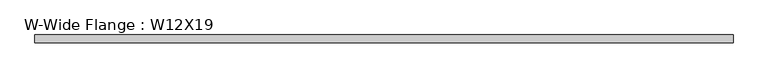
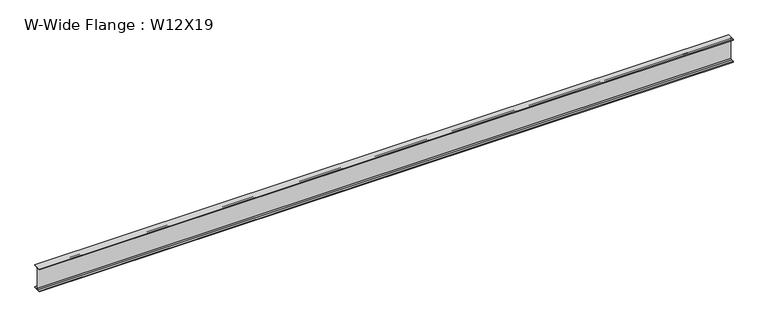
"""IFC4 building model written with IfcOpenShell, lengths in millimetres: beam geometry, W-Wide Flange : W12X19."""

import ifcopenshell
import ifcopenshell.guid

model = None  # the IFC model being written
_history = None  # IfcOwnerHistory: only IFC2X3 demands one
_inside = {}  # id of a spatial element -> (the spatial element, [elements in it])
_under = {}  # id of a project, library or spatial element -> (it, [spatial elements below it])
_declared = {}  # id of a project -> (the project, [libraries it declares])
_typed = {}  # id of a type object -> (the type object, [elements of that type])
_made_of = {}  # id of a material, layer set ... -> (it, [elements and type objects made of it])


def new_model(schema):
    """Start an empty IFC model of exactly this schema.

    Asked for "IFC4X3", IfcOpenShell would pick the latest addendum, in which some entities
    have other attributes; the version numbers below select the first issue.
    IFC2X3 requires an IfcOwnerHistory on every rooted entity: one is made here for all.
    """
    global model, _history
    if schema == "IFC4X3":
        model = ifcopenshell.file(schema_version=(4, 3, 0, 0))
    else:
        model = ifcopenshell.file(schema=schema)
    _inside.clear()
    _under.clear()
    _declared.clear()
    _typed.clear()
    _made_of.clear()
    _history = None
    if model.schema == "IFC2X3":
        org = make("IfcOrganization", Name="unknown")
        user = make(
            "IfcPersonAndOrganization",
            ThePerson=make("IfcPerson", FamilyName="unknown"),
            TheOrganization=org,
        )
        app = make(
            "IfcApplication",
            ApplicationDeveloper=org,
            Version="unknown",
            ApplicationFullName="unknown",
            ApplicationIdentifier="unknown",
        )
        _history = make(
            "IfcOwnerHistory",
            OwningUser=user,
            OwningApplication=app,
            ChangeAction="ADDED",
            CreationDate=0,
        )
    return model


def make(cls, **values):
    """One entity of the class cls with the attributes given. An attribute that is None is left unset."""
    return model.create_entity(
        cls, **{name: value for name, value in values.items() if value is not None}
    )


def rooted(cls, **values):
    """An entity with a GlobalId (a new one), such as an element, a storey or a relation."""
    return make(cls, GlobalId=ifcopenshell.guid.new(), OwnerHistory=_history, **values)


def si_unit(unit_type, name, prefix=None):
    """IfcSIUnit, for example si_unit("LENGTHUNIT", "METRE", prefix="MILLI")."""
    return make("IfcSIUnit", UnitType=unit_type, Prefix=prefix, Name=name)


def assignment(units):
    """IfcUnitAssignment: the units of a project."""
    return None if units is None else make("IfcUnitAssignment", Units=units)


def point(xyz):
    """IfcCartesianPoint."""
    return None if xyz is None else make("IfcCartesianPoint", Coordinates=xyz)


def direction(xyz):
    """IfcDirection."""
    return None if xyz is None else make("IfcDirection", DirectionRatios=xyz)


def frame(location, z_axis=None, x_axis=None):
    """IfcAxis2Placement3D, a coordinate frame: its origin and axes. An axis left out is left unset."""
    return make(
        "IfcAxis2Placement3D",
        Location=point(location),
        Axis=direction(z_axis),
        RefDirection=direction(x_axis),
    )


def frame_2d(location, x_axis=None):
    """IfcAxis2Placement2D, a coordinate frame in the plane: its origin and x axis."""
    return make(
        "IfcAxis2Placement2D", Location=point(location), RefDirection=direction(x_axis)
    )


def origin():
    """The frame at (0, 0, 0) with its axes left unset."""
    return frame((0.0, 0.0, 0.0))


def place(relative_to, where):
    """IfcLocalPlacement: puts the frame where relative to a parent placement (None: the world)."""
    return make(
        "IfcLocalPlacement", PlacementRelTo=relative_to, RelativePlacement=where
    )


def context(
    kind, dimensions, precision=None, world=None, true_north=None, identifier=None
):
    """IfcGeometricRepresentationContext, for example the 3D "Model" context."""
    return make(
        "IfcGeometricRepresentationContext",
        ContextIdentifier=identifier,
        ContextType=kind,
        CoordinateSpaceDimension=dimensions,
        Precision=precision,
        WorldCoordinateSystem=world,
        TrueNorth=true_north,
    )


def project(units=None, contexts=None):
    """IfcProject with its units and contexts."""
    return rooted(
        "IfcProject",
        Name="project",
        RepresentationContexts=contexts,
        UnitsInContext=assignment(units),
    )


def spatial(cls, under=None, at=None, **own):
    """A site, building, storey or space (cls), placed at a placement, below another one or the project."""
    s = rooted(cls, ObjectPlacement=at, **own)
    if under is not None:
        _under.setdefault(under.id(), (under, []))[1].append(s)
    return s


def polyline(points):
    """IfcPolyline through the points."""
    return make("IfcPolyline", Points=[point(p) for p in points])


def circle_curve(where, radius):
    """IfcCircle in the frame where."""
    return make("IfcCircle", Position=where, Radius=radius)


def trimmed(basis, trim1, trim2, sense, master):
    """IfcTrimmedCurve: the piece of a basis curve between two trims."""
    return make(
        "IfcTrimmedCurve",
        BasisCurve=basis,
        Trim1=trim1,
        Trim2=trim2,
        SenseAgreement=sense,
        MasterRepresentation=master,
    )


def segment(curve, same_sense, transition):
    """IfcCompositeCurveSegment."""
    return make(
        "IfcCompositeCurveSegment",
        Transition=transition,
        SameSense=same_sense,
        ParentCurve=curve,
    )


def composite_curve(segments, self_intersect=None):
    """IfcCompositeCurve: segments joined end to end."""
    return make("IfcCompositeCurve", Segments=segments, SelfIntersect=self_intersect)


def outline(outer, holes=None, kind="AREA"):
    """IfcArbitraryClosedProfileDef: a profile drawn as a closed curve; with holes, ...WithVoids."""
    if holes is None:
        return make("IfcArbitraryClosedProfileDef", ProfileType=kind, OuterCurve=outer)
    return make(
        "IfcArbitraryProfileDefWithVoids",
        ProfileType=kind,
        OuterCurve=outer,
        InnerCurves=holes,
    )


def extrude(swept, where, along, depth):
    """IfcExtrudedAreaSolid: the profile swept, set in the frame where, extruded along a direction by depth."""
    return make(
        "IfcExtrudedAreaSolid",
        SweptArea=swept,
        Position=where,
        ExtrudedDirection=direction(along),
        Depth=depth,
    )


def shape(context_of_items, identifier, shape_type, items):
    """IfcShapeRepresentation: the items that make up one representation, for example the "Body"."""
    return make(
        "IfcShapeRepresentation",
        ContextOfItems=context_of_items,
        RepresentationIdentifier=identifier,
        RepresentationType=shape_type,
        Items=items,
    )


def source(mapping_origin, context_of_items, identifier, shape_type, items):
    """IfcRepresentationMap: a shape defined once, which mapped items show again and again."""
    return make(
        "IfcRepresentationMap",
        MappingOrigin=mapping_origin,
        MappedRepresentation=shape(context_of_items, identifier, shape_type, items),
    )


def transform(
    local_origin,
    x_axis=None,
    y_axis=None,
    z_axis=None,
    scale=None,
    scale2=None,
    scale3=None,
    uniform=True,
):
    """IfcCartesianTransformationOperator3D, or its non-uniform kind. x_axis, y_axis, z_axis: its Axis1, 2, 3."""
    if uniform:
        return make(
            "IfcCartesianTransformationOperator3D",
            Axis1=direction(x_axis),
            Axis2=direction(y_axis),
            LocalOrigin=point(local_origin),
            Scale=scale,
            Axis3=direction(z_axis),
        )
    return make(
        "IfcCartesianTransformationOperator3DnonUniform",
        Axis1=direction(x_axis),
        Axis2=direction(y_axis),
        LocalOrigin=point(local_origin),
        Scale=scale,
        Axis3=direction(z_axis),
        Scale2=scale2,
        Scale3=scale3,
    )


def mapped(mapping_source, mapping_target):
    """IfcMappedItem: shows the shape of a source again, moved by a transform."""
    return make(
        "IfcMappedItem", MappingSource=mapping_source, MappingTarget=mapping_target
    )


def made_of(thing, what):
    """Note that an element or type object is made of a material, layer set ...; save() writes the relation."""
    if what is not None:
        _made_of.setdefault(what.id(), (what, []))[1].append(thing)
    return thing


def element(
    cls,
    number,
    at=None,
    inside=None,
    cuts=None,
    type_object=None,
    material=None,
    context=None,
    identifier="Body",
    shape_type=None,
    held_by="IfcProductDefinitionShape",
    body=None,
    shapes=None,
    **own,
):
    """One element of the class cls, such as IfcWall. Its Tag is "e" and its number.

    at: its placement. inside: the storey or other place that contains it. cuts: it is an
    opening in that element (IfcRelVoidsElement). A single representation is given by context,
    identifier, shape_type and body (its items); several are given by shapes. held_by: the class
    of the entity that holds the representations. save() writes the other relations.
    """
    e = rooted(cls, Tag="e%d" % number, ObjectPlacement=at, **own)
    if body is not None:
        shapes = [shape(context, identifier, shape_type, body)]
    if shapes is not None:
        e.Representation = make(held_by, Representations=shapes)
    if inside is not None:
        _inside.setdefault(inside.id(), (inside, []))[1].append(e)
    if cuts is not None:
        rooted(
            "IfcRelVoidsElement", RelatingBuildingElement=cuts, RelatedOpeningElement=e
        )
    if type_object is not None:
        _typed.setdefault(type_object.id(), (type_object, []))[1].append(e)
    return made_of(e, material)


def aggregate(whole, parts):
    """IfcRelAggregates: a whole, such as a stair, and the parts it consists of."""
    return rooted("IfcRelAggregates", RelatingObject=whole, RelatedObjects=parts)


def save(model, path):
    """Write the relations noted so far, then the file.

    IfcRelAggregates (storeys below a building ...), IfcRelContainedInSpatialStructure (elements
    in a storey), IfcRelDefinesByType, IfcRelAssociatesMaterial and IfcRelDeclares: one each for
    every whole, place, type object, material and project.
    """
    for whole, parts in _under.values():
        aggregate(whole, parts)
    for where, things in _inside.values():
        rooted(
            "IfcRelContainedInSpatialStructure",
            RelatedElements=things,
            RelatingStructure=where,
        )
    for kind, things in _typed.values():
        rooted("IfcRelDefinesByType", RelatedObjects=things, RelatingType=kind)
    for what, things in _made_of.values():
        rooted("IfcRelAssociatesMaterial", RelatedObjects=things, RelatingMaterial=what)
    for by, libraries in _declared.values():
        rooted("IfcRelDeclares", RelatingContext=by, RelatedDefinitions=libraries)
    model.write(path)


def w_wide_flange_w12x19_d63bb9e0(model_context):
    return source(origin(), model_context, "Body", "SweptSolid", [
        extrude(outline(composite_curve([segment(polyline([(50.927, -146.05), (50.927, -154.94), (-50.927, -154.94), (-50.927, -146.05), (-16.3195, -146.05)]), True, "CONTINUOUS"), segment(trimmed(circle_curve(frame_2d((-16.3195, -132.715)), 13.335), [point((-16.3195, -146.05))], [point((-2.9845, -132.715))], True, "CARTESIAN"), True, "CONTINUOUS"), segment(polyline([(-2.9845, -132.715), (-2.9845, 132.715)]), True, "CONTINUOUS"), segment(trimmed(circle_curve(frame_2d((-16.3195, 132.715)), 13.335), [point((-2.9845, 132.715))], [point((-16.3195, 146.05))], True, "CARTESIAN"), True, "CONTINUOUS"), segment(polyline([(-16.3195, 146.05), (-50.927, 146.05), (-50.927, 154.94), (50.927, 154.94), (50.927, 146.05), (16.3195, 146.05)]), True, "CONTINUOUS"), segment(trimmed(circle_curve(frame_2d((16.3195, 132.715)), 13.335), [point((16.3195, 146.05))], [point((2.9845, 132.715))], True, "CARTESIAN"), True, "CONTINUOUS"), segment(polyline([(2.9845, 132.715), (2.9845, -132.715)]), True, "CONTINUOUS"), segment(trimmed(circle_curve(frame_2d((16.3195, -132.715)), 13.335), [point((2.9845, -132.715))], [point((16.3195, -146.05))], True, "CARTESIAN"), True, "CONTINUOUS"), segment(polyline([(16.3195, -146.05), (50.927, -146.05)]), True, "CONTINUOUS")], self_intersect=False)), frame((-4381.4503906, 0.0, 0.0), z_axis=(1.0, 0.0, 0.0), x_axis=(0.0, 1.0, 0.0)), (0.0, 0.0, 1.0), 8953.4503906),
    ])


if __name__ == "__main__":
    model = new_model("IFC4")
    model_context = context("Model", 3, world=origin())
    ifc_project = project(units=[si_unit("LENGTHUNIT", "METRE", prefix="MILLI")], contexts=[model_context])
    site = spatial("IfcSite", under=ifc_project)
    building = spatial("IfcBuilding", under=site)
    placement = place(None, origin())
    w_wide_flange_w12x19_shape = w_wide_flange_w12x19_d63bb9e0(model_context)
    element("IfcBeam", 1, ObjectType="W-Wide Flange : W12X19", at=placement, inside=building, context=model_context, shape_type="MappedRepresentation", body=[
        mapped(w_wide_flange_w12x19_shape, transform((0.0, 0.0, 0.0), x_axis=(1.0, 0.0, 0.0), y_axis=(0.0, 1.0, 0.0), z_axis=(0.0, 0.0, 1.0))),
    ])
    save(model, "model.ifc")

# Revit data of these elements
# Type "W-Wide Flange : W12X19"
#   Assembly Code = "B10"
#   W = 19
#   Length [instance default] = 1524 mm
#   bf = 101.854 mm
#   d = 309.88 mm
#   k = 22.225 mm
#   k2 = 13.335 mm
#   tf = 8.89 mm
#   tw = 5.969 mm
#   A = 0.00359354 m²
#   Structural Material [instance default] = Steel ASTM A992
# Element 1 (IfcBeam, "W-Wide Flange : W12X19")
#   Structural Material = Aluminum, Anodized Red
#   Materials on its faces: "Aluminum, Anodized Red"
# Materials
#   "Steel ASTM A992": class "Metal", colour RGB 128 0 0, transparency 0, Description = "Structural steel 50ksi", Cost = 0
#   "Aluminum, Anodized Red": class "Metal", colour RGB 120 120 120, transparency 0, Description = "Anodized aluminum, red", Cost = 0
